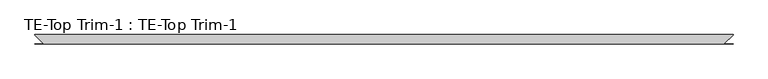
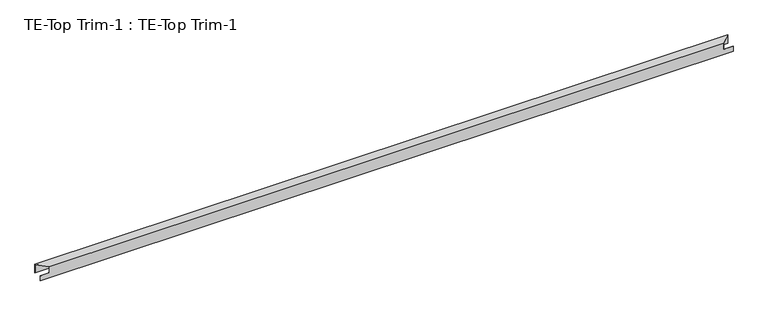
"""IFC4 building model written with IfcOpenShell, lengths in millimetres: proxy geometry, TE-Top Trim-1 : TE-Top Trim-1."""

import ifcopenshell
import ifcopenshell.guid

model = None  # the IFC model being written
_history = None  # IfcOwnerHistory: only IFC2X3 demands one
_inside = {}  # id of a spatial element -> (the spatial element, [elements in it])
_under = {}  # id of a project, library or spatial element -> (it, [spatial elements below it])
_declared = {}  # id of a project -> (the project, [libraries it declares])
_typed = {}  # id of a type object -> (the type object, [elements of that type])
_made_of = {}  # id of a material, layer set ... -> (it, [elements and type objects made of it])


def new_model(schema):
    """Start an empty IFC model of exactly this schema.

    Asked for "IFC4X3", IfcOpenShell would pick the latest addendum, in which some entities
    have other attributes; the version numbers below select the first issue.
    IFC2X3 requires an IfcOwnerHistory on every rooted entity: one is made here for all.
    """
    global model, _history
    if schema == "IFC4X3":
        model = ifcopenshell.file(schema_version=(4, 3, 0, 0))
    else:
        model = ifcopenshell.file(schema=schema)
    _inside.clear()
    _under.clear()
    _declared.clear()
    _typed.clear()
    _made_of.clear()
    _history = None
    if model.schema == "IFC2X3":
        org = make("IfcOrganization", Name="unknown")
        user = make(
            "IfcPersonAndOrganization",
            ThePerson=make("IfcPerson", FamilyName="unknown"),
            TheOrganization=org,
        )
        app = make(
            "IfcApplication",
            ApplicationDeveloper=org,
            Version="unknown",
            ApplicationFullName="unknown",
            ApplicationIdentifier="unknown",
        )
        _history = make(
            "IfcOwnerHistory",
            OwningUser=user,
            OwningApplication=app,
            ChangeAction="ADDED",
            CreationDate=0,
        )
    return model


def make(cls, **values):
    """One entity of the class cls with the attributes given. An attribute that is None is left unset."""
    return model.create_entity(
        cls, **{name: value for name, value in values.items() if value is not None}
    )


def rooted(cls, **values):
    """An entity with a GlobalId (a new one), such as an element, a storey or a relation."""
    return make(cls, GlobalId=ifcopenshell.guid.new(), OwnerHistory=_history, **values)


def si_unit(unit_type, name, prefix=None):
    """IfcSIUnit, for example si_unit("LENGTHUNIT", "METRE", prefix="MILLI")."""
    return make("IfcSIUnit", UnitType=unit_type, Prefix=prefix, Name=name)


def assignment(units):
    """IfcUnitAssignment: the units of a project."""
    return None if units is None else make("IfcUnitAssignment", Units=units)


def point(xyz):
    """IfcCartesianPoint."""
    return None if xyz is None else make("IfcCartesianPoint", Coordinates=xyz)


def direction(xyz):
    """IfcDirection."""
    return None if xyz is None else make("IfcDirection", DirectionRatios=xyz)


def frame(location, z_axis=None, x_axis=None):
    """IfcAxis2Placement3D, a coordinate frame: its origin and axes. An axis left out is left unset."""
    return make(
        "IfcAxis2Placement3D",
        Location=point(location),
        Axis=direction(z_axis),
        RefDirection=direction(x_axis),
    )


def origin():
    """The frame at (0, 0, 0) with its axes left unset."""
    return frame((0.0, 0.0, 0.0))


def place(relative_to, where):
    """IfcLocalPlacement: puts the frame where relative to a parent placement (None: the world)."""
    return make(
        "IfcLocalPlacement", PlacementRelTo=relative_to, RelativePlacement=where
    )


def context(
    kind, dimensions, precision=None, world=None, true_north=None, identifier=None
):
    """IfcGeometricRepresentationContext, for example the 3D "Model" context."""
    return make(
        "IfcGeometricRepresentationContext",
        ContextIdentifier=identifier,
        ContextType=kind,
        CoordinateSpaceDimension=dimensions,
        Precision=precision,
        WorldCoordinateSystem=world,
        TrueNorth=true_north,
    )


def project(units=None, contexts=None):
    """IfcProject with its units and contexts."""
    return rooted(
        "IfcProject",
        Name="project",
        RepresentationContexts=contexts,
        UnitsInContext=assignment(units),
    )


def spatial(cls, under=None, at=None, **own):
    """A site, building, storey or space (cls), placed at a placement, below another one or the project."""
    s = rooted(cls, ObjectPlacement=at, **own)
    if under is not None:
        _under.setdefault(under.id(), (under, []))[1].append(s)
    return s


def faces_of(points, faces, orient=None, outer=None):
    """IfcFace entities. A face is a list of loops; a loop is a list of indices into points, from 0.

    orient and outer hold one flag for each loop. By default every Orientation is true, the
    first loop of a face is its IfcFaceOuterBound and the others are IfcFaceBound.
    """
    made = []
    for i, loops in enumerate(faces):
        bounds = []
        for j, loop in enumerate(loops):
            is_outer = j == 0 if outer is None else outer[i][j]
            bounds.append(
                make(
                    "IfcFaceOuterBound" if is_outer else "IfcFaceBound",
                    Bound=make("IfcPolyLoop", Polygon=[points[k] for k in loop]),
                    Orientation=True if orient is None else orient[i][j],
                )
            )
        made.append(make("IfcFace", Bounds=bounds))
    return made


def faceted_brep(points, faces, orient=None, outer=None, voids=None):
    """IfcFacetedBrep: a solid bounded by flat faces; with voids (closed shells), ...WithVoids."""
    shared = [point(p) for p in points]
    hull = make("IfcClosedShell", CfsFaces=faces_of(shared, faces, orient, outer))
    if voids is None:
        return make("IfcFacetedBrep", Outer=hull)
    return make(
        "IfcFacetedBrepWithVoids",
        Outer=hull,
        Voids=[
            make(cls, CfsFaces=faces_of(shared, fs, o, b)) for cls, fs, o, b in voids
        ],
    )


def shape(context_of_items, identifier, shape_type, items):
    """IfcShapeRepresentation: the items that make up one representation, for example the "Body"."""
    return make(
        "IfcShapeRepresentation",
        ContextOfItems=context_of_items,
        RepresentationIdentifier=identifier,
        RepresentationType=shape_type,
        Items=items,
    )


def source(mapping_origin, context_of_items, identifier, shape_type, items):
    """IfcRepresentationMap: a shape defined once, which mapped items show again and again."""
    return make(
        "IfcRepresentationMap",
        MappingOrigin=mapping_origin,
        MappedRepresentation=shape(context_of_items, identifier, shape_type, items),
    )


def transform(
    local_origin,
    x_axis=None,
    y_axis=None,
    z_axis=None,
    scale=None,
    scale2=None,
    scale3=None,
    uniform=True,
):
    """IfcCartesianTransformationOperator3D, or its non-uniform kind. x_axis, y_axis, z_axis: its Axis1, 2, 3."""
    if uniform:
        return make(
            "IfcCartesianTransformationOperator3D",
            Axis1=direction(x_axis),
            Axis2=direction(y_axis),
            LocalOrigin=point(local_origin),
            Scale=scale,
            Axis3=direction(z_axis),
        )
    return make(
        "IfcCartesianTransformationOperator3DnonUniform",
        Axis1=direction(x_axis),
        Axis2=direction(y_axis),
        LocalOrigin=point(local_origin),
        Scale=scale,
        Axis3=direction(z_axis),
        Scale2=scale2,
        Scale3=scale3,
    )


def mapped(mapping_source, mapping_target):
    """IfcMappedItem: shows the shape of a source again, moved by a transform."""
    return make(
        "IfcMappedItem", MappingSource=mapping_source, MappingTarget=mapping_target
    )


def made_of(thing, what):
    """Note that an element or type object is made of a material, layer set ...; save() writes the relation."""
    if what is not None:
        _made_of.setdefault(what.id(), (what, []))[1].append(thing)
    return thing


def element(
    cls,
    number,
    at=None,
    inside=None,
    cuts=None,
    type_object=None,
    material=None,
    context=None,
    identifier="Body",
    shape_type=None,
    held_by="IfcProductDefinitionShape",
    body=None,
    shapes=None,
    **own,
):
    """One element of the class cls, such as IfcWall. Its Tag is "e" and its number.

    at: its placement. inside: the storey or other place that contains it. cuts: it is an
    opening in that element (IfcRelVoidsElement). A single representation is given by context,
    identifier, shape_type and body (its items); several are given by shapes. held_by: the class
    of the entity that holds the representations. save() writes the other relations.
    """
    e = rooted(cls, Tag="e%d" % number, ObjectPlacement=at, **own)
    if body is not None:
        shapes = [shape(context, identifier, shape_type, body)]
    if shapes is not None:
        e.Representation = make(held_by, Representations=shapes)
    if inside is not None:
        _inside.setdefault(inside.id(), (inside, []))[1].append(e)
    if cuts is not None:
        rooted(
            "IfcRelVoidsElement", RelatingBuildingElement=cuts, RelatedOpeningElement=e
        )
    if type_object is not None:
        _typed.setdefault(type_object.id(), (type_object, []))[1].append(e)
    return made_of(e, material)


def aggregate(whole, parts):
    """IfcRelAggregates: a whole, such as a stair, and the parts it consists of."""
    return rooted("IfcRelAggregates", RelatingObject=whole, RelatedObjects=parts)


def save(model, path):
    """Write the relations noted so far, then the file.

    IfcRelAggregates (storeys below a building ...), IfcRelContainedInSpatialStructure (elements
    in a storey), IfcRelDefinesByType, IfcRelAssociatesMaterial and IfcRelDeclares: one each for
    every whole, place, type object, material and project.
    """
    for whole, parts in _under.values():
        aggregate(whole, parts)
    for where, things in _inside.values():
        rooted(
            "IfcRelContainedInSpatialStructure",
            RelatedElements=things,
            RelatingStructure=where,
        )
    for kind, things in _typed.values():
        rooted("IfcRelDefinesByType", RelatedObjects=things, RelatingType=kind)
    for what, things in _made_of.values():
        rooted("IfcRelAssociatesMaterial", RelatedObjects=things, RelatingMaterial=what)
    for by, libraries in _declared.values():
        rooted("IfcRelDeclares", RelatingContext=by, RelatedDefinitions=libraries)
    model.write(path)


def te_top_trim_1_te_top_trim_1_ce3f5671(model_context):
    return source(origin(), model_context, "Body", "Brep", [
        faceted_brep([(587327.7934739, -531640.1093528, 2387.6), (587327.7934739, -531641.0023216, 2387.6), (587327.7934739, -531641.0023216, 2411.4125), (587327.7934739, -531640.1093528, 2411.4125), (587327.7934739, -531599.3917241, 2439.2929688), (587327.7934739, -531599.3917241, 2400.3), (587327.7934739, -531600.3289841, 2400.3), (587327.7934739, -531600.3289841, 2438.4), (587327.7934739, -531601.1251169, 2438.4), (587327.7934739, -531601.1251169, 2439.2929688), (590392.4558739, -531600.3289841, 2400.3), (590392.4558739, -531599.3917241, 2400.3), (590392.4558739, -531599.3917241, 2439.2929688), (590392.4558739, -531600.3190424, 2439.2929688), (590392.4558739, -531600.3190424, 2438.4), (590392.4558739, -531600.3289841, 2411.4125), (590392.4558739, -531641.0023216, 2387.6), (590392.4558739, -531640.1093528, 2387.6), (590392.4558739, -531640.1093528, 2411.4125), (590392.4558739, -531641.0023216, 2411.4125), (590351.7725947, -531641.0023216, 2411.4125), (590351.7725947, -531641.0023216, 2439.2929688), (587367.6706786, -531641.0023216, 2439.2929688), (587367.6706786, -531641.0023216, 2411.4125), (590352.6655635, -531640.1093528, 2438.4), (587366.7777099, -531640.1093528, 2438.4), (587366.7777099, -531640.1093528, 2411.4125), (590352.6655635, -531640.1093528, 2411.4125)], [[[0, 1, 2, 3]], [[4, 5, 6, 7, 8, 9]], [[10, 11, 12, 13, 14, 15]], [[16, 17, 18, 19]], [[1, 0, 17, 16]], [[1, 16, 19, 20, 21, 22, 23, 2]], [[12, 4, 9, 22, 21, 13]], [[5, 4, 12, 11]], [[6, 5, 11, 10]], [[7, 6, 10, 15, 14]], [[7, 14, 24, 25, 8]], [[17, 0, 3, 26, 25, 24, 27, 18]], [[27, 20, 19, 18]], [[20, 27, 24, 14, 13, 21]], [[23, 26, 3, 2]], [[26, 23, 22, 9, 8, 25]]]),
    ])


if __name__ == "__main__":
    model = new_model("IFC4")
    model_context = context("Model", 3, world=origin())
    ifc_project = project(units=[si_unit("LENGTHUNIT", "METRE", prefix="MILLI")], contexts=[model_context])
    site = spatial("IfcSite", under=ifc_project)
    building = spatial("IfcBuilding", under=site)
    placement = place(None, origin())
    te_top_trim_1_te_top_trim_1_shape = te_top_trim_1_te_top_trim_1_ce3f5671(model_context)
    element("IfcBuildingElementProxy", 1, Name="TE-Top Trim-1 : TE-Top Trim-1", ObjectType="TE-Top Trim-1 : TE-Top Trim-1", at=placement, inside=building, context=model_context, shape_type="MappedRepresentation", body=[
        mapped(te_top_trim_1_te_top_trim_1_shape, transform((0.0, 0.0, 0.0), x_axis=(1.0, 0.0, 0.0), y_axis=(0.0, 1.0, 0.0), z_axis=(0.0, 0.0, 1.0))),
    ])
    save(model, "model.ifc")

# Revit data of these elements
# Element 1 (IfcBuildingElementProxy, "TE-Top Trim-1 : TE-Top Trim-1")
#   Materials on its faces: "EDGE TRIM BY MTL PANEL MFR."
# Materials
#   "EDGE TRIM BY MTL PANEL MFR.": class "Generic", colour RGB 239 242 240, transparency 0, Cost = 0
